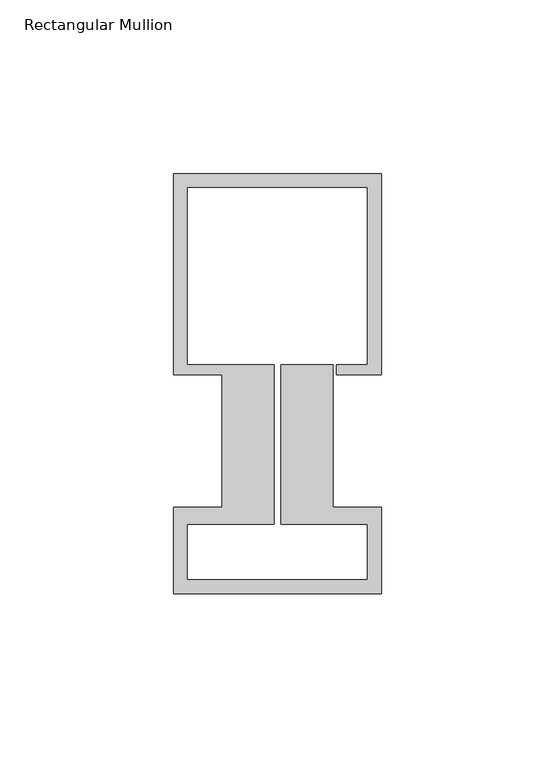
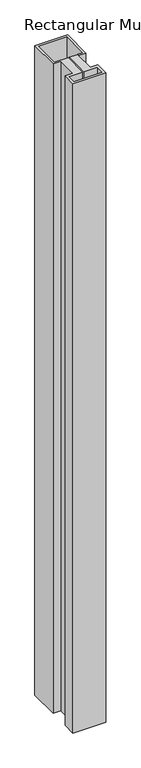
"""IFC4 building model written with IfcOpenShell, lengths in millimetres: member geometry, Rectangular Mullion : Schueco_FWS-60-SI_Tran_CovCap-20mm_Tran-55mm."""

import ifcopenshell
import ifcopenshell.guid

model = None  # the IFC model being written
_history = None  # IfcOwnerHistory: only IFC2X3 demands one
_inside = {}  # id of a spatial element -> (the spatial element, [elements in it])
_under = {}  # id of a project, library or spatial element -> (it, [spatial elements below it])
_declared = {}  # id of a project -> (the project, [libraries it declares])
_typed = {}  # id of a type object -> (the type object, [elements of that type])
_made_of = {}  # id of a material, layer set ... -> (it, [elements and type objects made of it])


def new_model(schema):
    """Start an empty IFC model of exactly this schema.

    Asked for "IFC4X3", IfcOpenShell would pick the latest addendum, in which some entities
    have other attributes; the version numbers below select the first issue.
    IFC2X3 requires an IfcOwnerHistory on every rooted entity: one is made here for all.
    """
    global model, _history
    if schema == "IFC4X3":
        model = ifcopenshell.file(schema_version=(4, 3, 0, 0))
    else:
        model = ifcopenshell.file(schema=schema)
    _inside.clear()
    _under.clear()
    _declared.clear()
    _typed.clear()
    _made_of.clear()
    _history = None
    if model.schema == "IFC2X3":
        org = make("IfcOrganization", Name="unknown")
        user = make(
            "IfcPersonAndOrganization",
            ThePerson=make("IfcPerson", FamilyName="unknown"),
            TheOrganization=org,
        )
        app = make(
            "IfcApplication",
            ApplicationDeveloper=org,
            Version="unknown",
            ApplicationFullName="unknown",
            ApplicationIdentifier="unknown",
        )
        _history = make(
            "IfcOwnerHistory",
            OwningUser=user,
            OwningApplication=app,
            ChangeAction="ADDED",
            CreationDate=0,
        )
    return model


def make(cls, **values):
    """One entity of the class cls with the attributes given. An attribute that is None is left unset."""
    return model.create_entity(
        cls, **{name: value for name, value in values.items() if value is not None}
    )


def rooted(cls, **values):
    """An entity with a GlobalId (a new one), such as an element, a storey or a relation."""
    return make(cls, GlobalId=ifcopenshell.guid.new(), OwnerHistory=_history, **values)


def si_unit(unit_type, name, prefix=None):
    """IfcSIUnit, for example si_unit("LENGTHUNIT", "METRE", prefix="MILLI")."""
    return make("IfcSIUnit", UnitType=unit_type, Prefix=prefix, Name=name)


def assignment(units):
    """IfcUnitAssignment: the units of a project."""
    return None if units is None else make("IfcUnitAssignment", Units=units)


def point(xyz):
    """IfcCartesianPoint."""
    return None if xyz is None else make("IfcCartesianPoint", Coordinates=xyz)


def direction(xyz):
    """IfcDirection."""
    return None if xyz is None else make("IfcDirection", DirectionRatios=xyz)


def frame(location, z_axis=None, x_axis=None):
    """IfcAxis2Placement3D, a coordinate frame: its origin and axes. An axis left out is left unset."""
    return make(
        "IfcAxis2Placement3D",
        Location=point(location),
        Axis=direction(z_axis),
        RefDirection=direction(x_axis),
    )


def origin():
    """The frame at (0, 0, 0) with its axes left unset."""
    return frame((0.0, 0.0, 0.0))


def place(relative_to, where):
    """IfcLocalPlacement: puts the frame where relative to a parent placement (None: the world)."""
    return make(
        "IfcLocalPlacement", PlacementRelTo=relative_to, RelativePlacement=where
    )


def context(
    kind, dimensions, precision=None, world=None, true_north=None, identifier=None
):
    """IfcGeometricRepresentationContext, for example the 3D "Model" context."""
    return make(
        "IfcGeometricRepresentationContext",
        ContextIdentifier=identifier,
        ContextType=kind,
        CoordinateSpaceDimension=dimensions,
        Precision=precision,
        WorldCoordinateSystem=world,
        TrueNorth=true_north,
    )


def project(units=None, contexts=None):
    """IfcProject with its units and contexts."""
    return rooted(
        "IfcProject",
        Name="project",
        RepresentationContexts=contexts,
        UnitsInContext=assignment(units),
    )


def spatial(cls, under=None, at=None, **own):
    """A site, building, storey or space (cls), placed at a placement, below another one or the project."""
    s = rooted(cls, ObjectPlacement=at, **own)
    if under is not None:
        _under.setdefault(under.id(), (under, []))[1].append(s)
    return s


def polyline(points):
    """IfcPolyline through the points."""
    return make("IfcPolyline", Points=[point(p) for p in points])


def outline(outer, holes=None, kind="AREA"):
    """IfcArbitraryClosedProfileDef: a profile drawn as a closed curve; with holes, ...WithVoids."""
    if holes is None:
        return make("IfcArbitraryClosedProfileDef", ProfileType=kind, OuterCurve=outer)
    return make(
        "IfcArbitraryProfileDefWithVoids",
        ProfileType=kind,
        OuterCurve=outer,
        InnerCurves=holes,
    )


def extrude(swept, where, along, depth):
    """IfcExtrudedAreaSolid: the profile swept, set in the frame where, extruded along a direction by depth."""
    return make(
        "IfcExtrudedAreaSolid",
        SweptArea=swept,
        Position=where,
        ExtrudedDirection=direction(along),
        Depth=depth,
    )


def shape(context_of_items, identifier, shape_type, items):
    """IfcShapeRepresentation: the items that make up one representation, for example the "Body"."""
    return make(
        "IfcShapeRepresentation",
        ContextOfItems=context_of_items,
        RepresentationIdentifier=identifier,
        RepresentationType=shape_type,
        Items=items,
    )


def source(mapping_origin, context_of_items, identifier, shape_type, items):
    """IfcRepresentationMap: a shape defined once, which mapped items show again and again."""
    return make(
        "IfcRepresentationMap",
        MappingOrigin=mapping_origin,
        MappedRepresentation=shape(context_of_items, identifier, shape_type, items),
    )


def transform(
    local_origin,
    x_axis=None,
    y_axis=None,
    z_axis=None,
    scale=None,
    scale2=None,
    scale3=None,
    uniform=True,
):
    """IfcCartesianTransformationOperator3D, or its non-uniform kind. x_axis, y_axis, z_axis: its Axis1, 2, 3."""
    if uniform:
        return make(
            "IfcCartesianTransformationOperator3D",
            Axis1=direction(x_axis),
            Axis2=direction(y_axis),
            LocalOrigin=point(local_origin),
            Scale=scale,
            Axis3=direction(z_axis),
        )
    return make(
        "IfcCartesianTransformationOperator3DnonUniform",
        Axis1=direction(x_axis),
        Axis2=direction(y_axis),
        LocalOrigin=point(local_origin),
        Scale=scale,
        Axis3=direction(z_axis),
        Scale2=scale2,
        Scale3=scale3,
    )


def mapped(mapping_source, mapping_target):
    """IfcMappedItem: shows the shape of a source again, moved by a transform."""
    return make(
        "IfcMappedItem", MappingSource=mapping_source, MappingTarget=mapping_target
    )


def made_of(thing, what):
    """Note that an element or type object is made of a material, layer set ...; save() writes the relation."""
    if what is not None:
        _made_of.setdefault(what.id(), (what, []))[1].append(thing)
    return thing


def element(
    cls,
    number,
    at=None,
    inside=None,
    cuts=None,
    type_object=None,
    material=None,
    context=None,
    identifier="Body",
    shape_type=None,
    held_by="IfcProductDefinitionShape",
    body=None,
    shapes=None,
    **own,
):
    """One element of the class cls, such as IfcWall. Its Tag is "e" and its number.

    at: its placement. inside: the storey or other place that contains it. cuts: it is an
    opening in that element (IfcRelVoidsElement). A single representation is given by context,
    identifier, shape_type and body (its items); several are given by shapes. held_by: the class
    of the entity that holds the representations. save() writes the other relations.
    """
    e = rooted(cls, Tag="e%d" % number, ObjectPlacement=at, **own)
    if body is not None:
        shapes = [shape(context, identifier, shape_type, body)]
    if shapes is not None:
        e.Representation = make(held_by, Representations=shapes)
    if inside is not None:
        _inside.setdefault(inside.id(), (inside, []))[1].append(e)
    if cuts is not None:
        rooted(
            "IfcRelVoidsElement", RelatingBuildingElement=cuts, RelatedOpeningElement=e
        )
    if type_object is not None:
        _typed.setdefault(type_object.id(), (type_object, []))[1].append(e)
    return made_of(e, material)


def aggregate(whole, parts):
    """IfcRelAggregates: a whole, such as a stair, and the parts it consists of."""
    return rooted("IfcRelAggregates", RelatingObject=whole, RelatedObjects=parts)


def save(model, path):
    """Write the relations noted so far, then the file.

    IfcRelAggregates (storeys below a building ...), IfcRelContainedInSpatialStructure (elements
    in a storey), IfcRelDefinesByType, IfcRelAssociatesMaterial and IfcRelDeclares: one each for
    every whole, place, type object, material and project.
    """
    for whole, parts in _under.values():
        aggregate(whole, parts)
    for where, things in _inside.values():
        rooted(
            "IfcRelContainedInSpatialStructure",
            RelatedElements=things,
            RelatingStructure=where,
        )
    for kind, things in _typed.values():
        rooted("IfcRelDefinesByType", RelatedObjects=things, RelatingType=kind)
    for what, things in _made_of.values():
        rooted("IfcRelAssociatesMaterial", RelatedObjects=things, RelatingMaterial=what)
    for by, libraries in _declared.values():
        rooted("IfcRelDeclares", RelatingContext=by, RelatedDefinitions=libraries)
    model.write(path)


def rectangular_mullion_714c4c15(model_context):
    return source(origin(), model_context, "Body", "SweptSolid", [
        extrude(outline(polyline([(-60.0, 96.0), (0.0, 96.0), (0.0, 38.0), (-13.0, 38.0), (-13.0, 41.0), (-4.0, 41.0), (-4.0, 92.0), (-56.0, 92.0), (-56.0, 41.0), (-31.0, 41.0), (-31.0, -5.0), (-56.0, -5.0), (-56.0, -21.0), (-4.0, -21.0), (-4.0, -5.0), (-29.0, -5.0), (-29.0, 41.0), (-14.0, 41.0), (-14.0, -0.1), (0.0, -0.1), (0.0, -25.0), (-60.0, -25.0), (-60.0, -0.1), (-46.0, -0.1), (-46.0, 38.0), (-60.0, 38.0), (-60.0, 96.0)])), frame((0.0, 0.0, -1260.0), z_axis=(0.0, 0.0, 1.0), x_axis=(1.0, 0.0, 0.0)), (0.0, 0.0, 1.0), 1260.0),
    ])


if __name__ == "__main__":
    model = new_model("IFC4")
    model_context = context("Model", 3, world=origin())
    ifc_project = project(units=[si_unit("LENGTHUNIT", "METRE", prefix="MILLI")], contexts=[model_context])
    site = spatial("IfcSite", under=ifc_project)
    building = spatial("IfcBuilding", under=site)
    placement = place(None, origin())
    rectangular_mullion_shape = rectangular_mullion_714c4c15(model_context)
    element("IfcMember", 1, ObjectType="Rectangular Mullion : Schueco_FWS-60-SI_Tran_CovCap-20mm_Tran-55mm", at=placement, inside=building, context=model_context, shape_type="MappedRepresentation", body=[
        mapped(rectangular_mullion_shape, transform((0.0, 0.0, 0.0), x_axis=(1.0, 0.0, 0.0), y_axis=(0.0, 1.0, 0.0), z_axis=(0.0, 0.0, 1.0))),
    ])
    save(model, "model.ifc")

# Revit data of these elements
# Type "Rectangular Mullion : Schueco_FWS-60-SI_Tran_CovCap-20mm_Tran-55mm"
#   Model = "FWS 60.SI"
#   Manufacturer = "Schueco International KG"
#   Type Comments = "Transom"
#   Schueco thermal insulation standard = "Suitable for passive houses"
#   Burglar resistance = "RC 3"
#   Thermal insulation = "to 0.70 W/(m²K)"
#   built-in parameter 1007322 = 0.396982 (stored number, unit not read)
#   built-in parameter 1007321 = 0.0524934 (stored number, unit not read)
#   built-in parameter 1007320 = 0.0524934 (stored number, unit not read)
# Element 1 (IfcMember, "Rectangular Mullion : Schueco_FWS-60-SI_Tran_CovCap-20mm_Tran-55mm")
#   Materials on its faces: "Alu"
# Materials
#   "Alu": class "Glas", colour RGB 140 140 140, transparency 0
